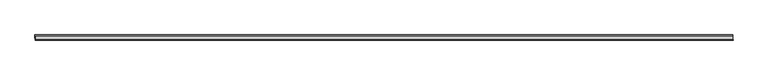
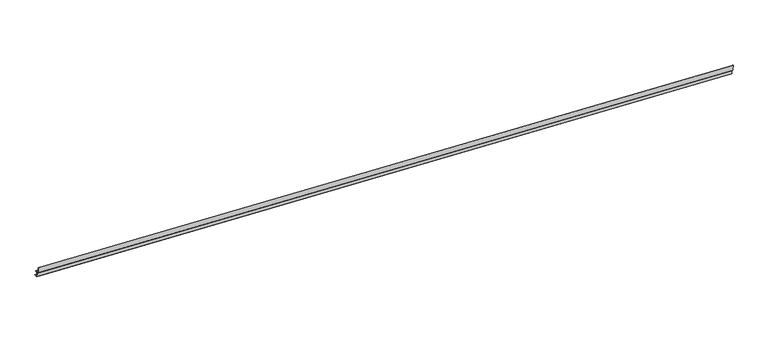
"""IFC4 building model written with IfcOpenShell, lengths in millimetres: proxy geometry, Generic Models 2:Generic Models 2:310765:Generic Models 2:310765 : Generic Models 2:Generic Models 2:310765:194 : Generic Models 2:Generic Models 2:310765:Generic Models 2:310765 : Generic Models 2:Generic Models 2:310765:300385."""

from ifc_helpers import new_model, si_unit, frame, origin, place, context, project, spatial, polyline, outline, extrude, source, transform, mapped, element, save


def generic_models_47019f70(model_context):
    return source(origin(), model_context, "Body", "SweptSolid", [
        extrude(outline(polyline([(146.05, 0.0), (146.05, -64.157564), (155.575, -64.157564), (155.575, -46.695064), (157.1625, -46.695064), (157.1625, -65.745064), (144.4625, -65.745064), (144.4625, -1.5875), (55.5625, -1.5875), (55.5625, 0.0), (146.05, 0.0)])), frame((800591.9511155, -578781.6163841, 4280.4506205), z_axis=(-0.9991330730923567, 0.0, 0.04163054471206784), x_axis=(-0.04163054471206784, 0.0, -0.9991330730923567)), (0.0, 0.0, 1.0), 12411.242059),
        extrude(outline(polyline([(151.60625, -42.3509311), (151.60625, -61.2200628), (150.01875, -61.2200628), (150.01875, -40.7634311), (202.40625, -40.7634311), (202.40625, -42.3509311), (151.60625, -42.3509311)])), frame((800591.9511155, -578781.6163841, 4280.4506205), z_axis=(-0.9991330730923567, 0.0, 0.04163054471206784), x_axis=(-0.04163054471206784, 0.0, -0.9991330730923567)), (0.0, 0.0, 1.0), 12411.242059),
        extrude(outline(polyline([(235.74375, -30.1625), (235.74375, -91.3825628), (234.15625, -91.3825628), (234.15625, -31.75), (172.24375, -31.75), (172.24375, -30.1625), (235.74375, -30.1625)])), frame((800591.9511155, -578781.6163841, 4280.4506205), z_axis=(-0.9991330730923567, 0.0, 0.04163054471206784), x_axis=(-0.04163054471206784, 0.0, -0.9991330730923567)), (0.0, 0.0, 1.0), 12411.242059),
    ])


if __name__ == "__main__":
    model = new_model("IFC4")
    model_context = context("Model", 3, world=origin())
    ifc_project = project(units=[si_unit("LENGTHUNIT", "METRE", prefix="MILLI")], contexts=[model_context])
    site = spatial("IfcSite", under=ifc_project)
    building = spatial("IfcBuilding", under=site)
    placement = place(None, origin())
    generic_models_shape = generic_models_47019f70(model_context)
    element("IfcBuildingElementProxy", 1, Name="Generic Models 2:Generic Models 2:310765:Generic Models 2:310765 : Generic Models 2:Generic Models 2:310765:194 : Generic Models 2:Generic Models 2:310765:Generic Models 2:310765 : Generic Models 2:Generic Models 2:310765:300385", ObjectType="Generic Models 2:Generic Models 2:310765:Generic Models 2:310765 : Generic Models 2:Generic Models 2:310765:194 : Generic Models 2:Generic Models 2:310765:Generic Models 2:310765 : Generic Models 2:Generic Models 2:310765:300385", at=placement, inside=building, context=model_context, shape_type="MappedRepresentation", body=[
        mapped(generic_models_shape, transform((0.0, 0.0, 0.0), x_axis=(1.0, 0.0, 0.0), y_axis=(0.0, 1.0, 0.0), z_axis=(0.0, 0.0, 1.0))),
    ])
    save(model, "model.ifc")

# Revit data of these elements
# Type "Generic Models 2:Generic Models 2:310765:Generic Models 2:310765 : Generic Models 2:Generic Models 2:310765:194 : Generic Models 2:Generic Models 2:310765:Generic Models 2:310765 : Generic Models 2:Generic Models 2:310765:300385"
#   NameOverride = "Generic Models 2:Generic Models 2:310765:Generic Models 2:310765 : Generic Models 2:Generic Models 2:310765:300385"
#   ObjectTypeOverride = "Generic Models 2:310765 : Generic Models 2:Generic Models 2:310765"
#   Reference = "Generic Models 2"
#   Tag = "300385"
# Element 1 (IfcBuildingElementProxy, "Generic Models 2:Generic Models 2:310765:Generic Models 2:310765 : Generic Models 2:Generic Models 2:310765:194 : Generic Models 2:Generic Models 2:310765:Generic Models 2:310765 : Generic Models 2:Generic Models 2:310765:300385")
#   Materials on its faces: "BRAKE METAL COUNTERFLASHING"
# Materials
#   "BRAKE METAL COUNTERFLASHING": class "Unassigned", colour RGB 210 209 208, transparency 0, Cost = 0
